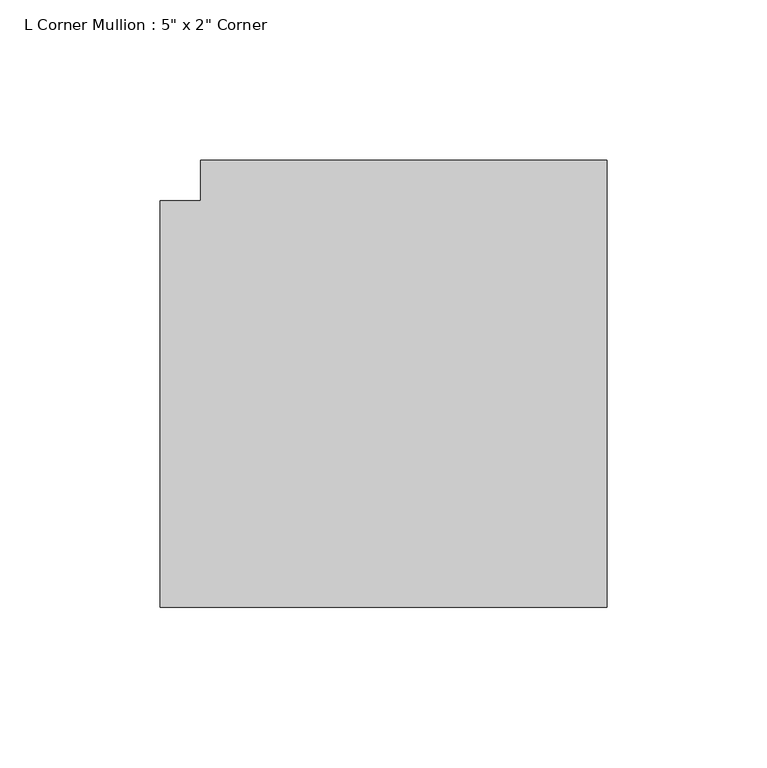
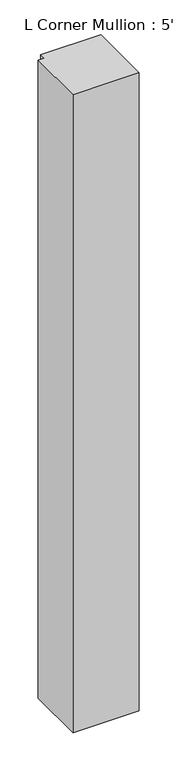
"""IFC4 building model written with IfcOpenShell, lengths in millimetres: member geometry."""

from ifc_helpers import new_model, si_unit, frame, origin, place, context, project, spatial, polyline, outline, extrude, source, transform, mapped, element, save


def member_a25f7c35(model_context):
    return source(origin(), model_context, "Body", "SweptSolid", [
        extrude(outline(polyline([(63.5, 76.2), (63.5, -63.5), (-76.2, -63.5), (-76.2, 63.5), (-63.5, 63.5), (-63.5, 76.2), (63.5, 76.2)])), frame((0.0, 0.0, -1422.4), z_axis=(0.0, 0.0, 1.0), x_axis=(1.0, 0.0, 0.0)), (0.0, 0.0, 1.0), 1422.4),
    ])


if __name__ == "__main__":
    model = new_model("IFC4")
    model_context = context("Model", 3, world=origin())
    ifc_project = project(units=[si_unit("LENGTHUNIT", "METRE", prefix="MILLI")], contexts=[model_context])
    site = spatial("IfcSite", under=ifc_project)
    building = spatial("IfcBuilding", under=site)
    placement = place(None, origin())
    member_shape = member_a25f7c35(model_context)
    element("IfcMember", 1, ObjectType="L Corner Mullion : 5\" x 2\" Corner", at=placement, inside=building, context=model_context, shape_type="MappedRepresentation", body=[
        mapped(member_shape, transform((0.0, 0.0, 0.0), x_axis=(1.0, 0.0, 0.0), y_axis=(0.0, 1.0, 0.0), z_axis=(0.0, 0.0, 1.0))),
    ])
    save(model, "model.ifc")

# Revit data of these elements
# Type "L Corner Mullion : 5\" x 2\" Corner"
#   built-in parameter 1007355 = 0.25 (stored number, unit not read)
#   built-in parameter 1007354 = 0.25 (stored number, unit not read)
#   built-in parameter 1007304 = 0.416667 (stored number, unit not read)
# Element 1 (IfcMember, "L Corner Mullion : 5\" x 2\" Corner")
#   Materials on its faces: "Metal - Aluminum"
# Materials
#   "Metal - Aluminum": class "Metal", colour RGB 109 108 108, transparency 0
